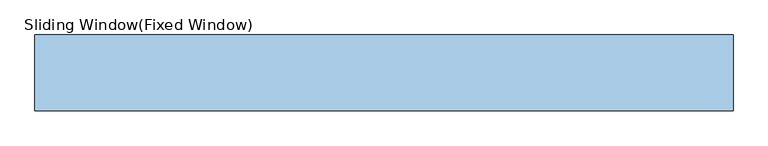
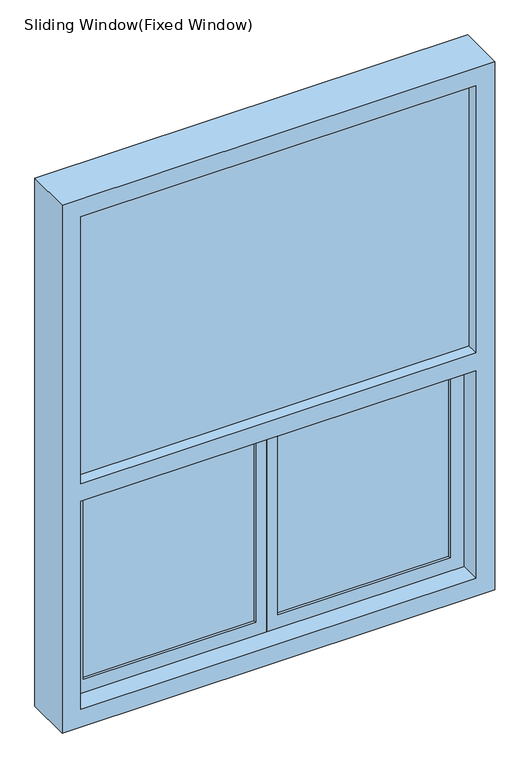
"""IFC4 building model written with IfcOpenShell, lengths in millimetres: window geometry, Sliding Window(Fixed Window) : H_WD_AR_B11_Fix_Sliding_Steel Window_DG_W1400xH1800_AW-1."""

import ifcopenshell
import ifcopenshell.guid

model = None  # the IFC model being written
_history = None  # IfcOwnerHistory: only IFC2X3 demands one
_inside = {}  # id of a spatial element -> (the spatial element, [elements in it])
_under = {}  # id of a project, library or spatial element -> (it, [spatial elements below it])
_declared = {}  # id of a project -> (the project, [libraries it declares])
_typed = {}  # id of a type object -> (the type object, [elements of that type])
_made_of = {}  # id of a material, layer set ... -> (it, [elements and type objects made of it])


def new_model(schema):
    """Start an empty IFC model of exactly this schema.

    Asked for "IFC4X3", IfcOpenShell would pick the latest addendum, in which some entities
    have other attributes; the version numbers below select the first issue.
    IFC2X3 requires an IfcOwnerHistory on every rooted entity: one is made here for all.
    """
    global model, _history
    if schema == "IFC4X3":
        model = ifcopenshell.file(schema_version=(4, 3, 0, 0))
    else:
        model = ifcopenshell.file(schema=schema)
    _inside.clear()
    _under.clear()
    _declared.clear()
    _typed.clear()
    _made_of.clear()
    _history = None
    if model.schema == "IFC2X3":
        org = make("IfcOrganization", Name="unknown")
        user = make(
            "IfcPersonAndOrganization",
            ThePerson=make("IfcPerson", FamilyName="unknown"),
            TheOrganization=org,
        )
        app = make(
            "IfcApplication",
            ApplicationDeveloper=org,
            Version="unknown",
            ApplicationFullName="unknown",
            ApplicationIdentifier="unknown",
        )
        _history = make(
            "IfcOwnerHistory",
            OwningUser=user,
            OwningApplication=app,
            ChangeAction="ADDED",
            CreationDate=0,
        )
    return model


def make(cls, **values):
    """One entity of the class cls with the attributes given. An attribute that is None is left unset."""
    return model.create_entity(
        cls, **{name: value for name, value in values.items() if value is not None}
    )


def rooted(cls, **values):
    """An entity with a GlobalId (a new one), such as an element, a storey or a relation."""
    return make(cls, GlobalId=ifcopenshell.guid.new(), OwnerHistory=_history, **values)


def si_unit(unit_type, name, prefix=None):
    """IfcSIUnit, for example si_unit("LENGTHUNIT", "METRE", prefix="MILLI")."""
    return make("IfcSIUnit", UnitType=unit_type, Prefix=prefix, Name=name)


def assignment(units):
    """IfcUnitAssignment: the units of a project."""
    return None if units is None else make("IfcUnitAssignment", Units=units)


def point(xyz):
    """IfcCartesianPoint."""
    return None if xyz is None else make("IfcCartesianPoint", Coordinates=xyz)


def direction(xyz):
    """IfcDirection."""
    return None if xyz is None else make("IfcDirection", DirectionRatios=xyz)


def frame(location, z_axis=None, x_axis=None):
    """IfcAxis2Placement3D, a coordinate frame: its origin and axes. An axis left out is left unset."""
    return make(
        "IfcAxis2Placement3D",
        Location=point(location),
        Axis=direction(z_axis),
        RefDirection=direction(x_axis),
    )


def origin():
    """The frame at (0, 0, 0) with its axes left unset."""
    return frame((0.0, 0.0, 0.0))


def place(relative_to, where):
    """IfcLocalPlacement: puts the frame where relative to a parent placement (None: the world)."""
    return make(
        "IfcLocalPlacement", PlacementRelTo=relative_to, RelativePlacement=where
    )


def context(
    kind, dimensions, precision=None, world=None, true_north=None, identifier=None
):
    """IfcGeometricRepresentationContext, for example the 3D "Model" context."""
    return make(
        "IfcGeometricRepresentationContext",
        ContextIdentifier=identifier,
        ContextType=kind,
        CoordinateSpaceDimension=dimensions,
        Precision=precision,
        WorldCoordinateSystem=world,
        TrueNorth=true_north,
    )


def project(units=None, contexts=None):
    """IfcProject with its units and contexts."""
    return rooted(
        "IfcProject",
        Name="project",
        RepresentationContexts=contexts,
        UnitsInContext=assignment(units),
    )


def spatial(cls, under=None, at=None, **own):
    """A site, building, storey or space (cls), placed at a placement, below another one or the project."""
    s = rooted(cls, ObjectPlacement=at, **own)
    if under is not None:
        _under.setdefault(under.id(), (under, []))[1].append(s)
    return s


def polyline(points):
    """IfcPolyline through the points."""
    return make("IfcPolyline", Points=[point(p) for p in points])


def outline(outer, holes=None, kind="AREA"):
    """IfcArbitraryClosedProfileDef: a profile drawn as a closed curve; with holes, ...WithVoids."""
    if holes is None:
        return make("IfcArbitraryClosedProfileDef", ProfileType=kind, OuterCurve=outer)
    return make(
        "IfcArbitraryProfileDefWithVoids",
        ProfileType=kind,
        OuterCurve=outer,
        InnerCurves=holes,
    )


def extrude(swept, where, along, depth):
    """IfcExtrudedAreaSolid: the profile swept, set in the frame where, extruded along a direction by depth."""
    return make(
        "IfcExtrudedAreaSolid",
        SweptArea=swept,
        Position=where,
        ExtrudedDirection=direction(along),
        Depth=depth,
    )


def shape(context_of_items, identifier, shape_type, items):
    """IfcShapeRepresentation: the items that make up one representation, for example the "Body"."""
    return make(
        "IfcShapeRepresentation",
        ContextOfItems=context_of_items,
        RepresentationIdentifier=identifier,
        RepresentationType=shape_type,
        Items=items,
    )


def source(mapping_origin, context_of_items, identifier, shape_type, items):
    """IfcRepresentationMap: a shape defined once, which mapped items show again and again."""
    return make(
        "IfcRepresentationMap",
        MappingOrigin=mapping_origin,
        MappedRepresentation=shape(context_of_items, identifier, shape_type, items),
    )


def transform(
    local_origin,
    x_axis=None,
    y_axis=None,
    z_axis=None,
    scale=None,
    scale2=None,
    scale3=None,
    uniform=True,
):
    """IfcCartesianTransformationOperator3D, or its non-uniform kind. x_axis, y_axis, z_axis: its Axis1, 2, 3."""
    if uniform:
        return make(
            "IfcCartesianTransformationOperator3D",
            Axis1=direction(x_axis),
            Axis2=direction(y_axis),
            LocalOrigin=point(local_origin),
            Scale=scale,
            Axis3=direction(z_axis),
        )
    return make(
        "IfcCartesianTransformationOperator3DnonUniform",
        Axis1=direction(x_axis),
        Axis2=direction(y_axis),
        LocalOrigin=point(local_origin),
        Scale=scale,
        Axis3=direction(z_axis),
        Scale2=scale2,
        Scale3=scale3,
    )


def mapped(mapping_source, mapping_target):
    """IfcMappedItem: shows the shape of a source again, moved by a transform."""
    return make(
        "IfcMappedItem", MappingSource=mapping_source, MappingTarget=mapping_target
    )


def made_of(thing, what):
    """Note that an element or type object is made of a material, layer set ...; save() writes the relation."""
    if what is not None:
        _made_of.setdefault(what.id(), (what, []))[1].append(thing)
    return thing


def element(
    cls,
    number,
    at=None,
    inside=None,
    cuts=None,
    type_object=None,
    material=None,
    context=None,
    identifier="Body",
    shape_type=None,
    held_by="IfcProductDefinitionShape",
    body=None,
    shapes=None,
    **own,
):
    """One element of the class cls, such as IfcWall. Its Tag is "e" and its number.

    at: its placement. inside: the storey or other place that contains it. cuts: it is an
    opening in that element (IfcRelVoidsElement). A single representation is given by context,
    identifier, shape_type and body (its items); several are given by shapes. held_by: the class
    of the entity that holds the representations. save() writes the other relations.
    """
    e = rooted(cls, Tag="e%d" % number, ObjectPlacement=at, **own)
    if body is not None:
        shapes = [shape(context, identifier, shape_type, body)]
    if shapes is not None:
        e.Representation = make(held_by, Representations=shapes)
    if inside is not None:
        _inside.setdefault(inside.id(), (inside, []))[1].append(e)
    if cuts is not None:
        rooted(
            "IfcRelVoidsElement", RelatingBuildingElement=cuts, RelatedOpeningElement=e
        )
    if type_object is not None:
        _typed.setdefault(type_object.id(), (type_object, []))[1].append(e)
    return made_of(e, material)


def aggregate(whole, parts):
    """IfcRelAggregates: a whole, such as a stair, and the parts it consists of."""
    return rooted("IfcRelAggregates", RelatingObject=whole, RelatedObjects=parts)


def save(model, path):
    """Write the relations noted so far, then the file.

    IfcRelAggregates (storeys below a building ...), IfcRelContainedInSpatialStructure (elements
    in a storey), IfcRelDefinesByType, IfcRelAssociatesMaterial and IfcRelDeclares: one each for
    every whole, place, type object, material and project.
    """
    for whole, parts in _under.values():
        aggregate(whole, parts)
    for where, things in _inside.values():
        rooted(
            "IfcRelContainedInSpatialStructure",
            RelatedElements=things,
            RelatingStructure=where,
        )
    for kind, things in _typed.values():
        rooted("IfcRelDefinesByType", RelatedObjects=things, RelatingType=kind)
    for what, things in _made_of.values():
        rooted("IfcRelAssociatesMaterial", RelatedObjects=things, RelatingMaterial=what)
    for by, libraries in _declared.values():
        rooted("IfcRelDeclares", RelatingContext=by, RelatedDefinitions=libraries)
    model.write(path)


def sliding_window_fixed_window_7f21aae4(model_context):
    return source(origin(), model_context, "Body", "SweptSolid", [
        extrude(outline(polyline([(2830.0, -690.0), (1050.0, -690.0), (1050.0, 690.0), (2830.0, 690.0), (2830.0, -690.0)]), holes=[polyline([(1810.0, 630.0), (1110.0, 630.0), (1110.0, -630.0), (1810.0, -630.0), (1810.0, 630.0)]), polyline([(1870.0, -630.0), (2770.0, -630.0), (2770.0, 630.0), (1870.0, 630.0), (1870.0, -630.0)])]), frame((0.0, -25.0, 0.0), z_axis=(0.0, 1.0, 0.0), x_axis=(0.0, 0.0, 1.0)), (0.0, 0.0, 1.0), 150.0),
        extrude(outline(polyline([(630.0, 37.0), (630.0, 13.0), (-630.0, 13.0), (-630.0, 37.0), (630.0, 37.0)])), frame((0.0, 0.0, 1870.0), z_axis=(0.0, 0.0, 1.0), x_axis=(1.0, 0.0, 0.0)), (0.0, 0.0, 1.0), 900.0),
        extrude(outline(polyline([(-35.0, 61.0), (-35.0, 49.0), (-585.0, 49.0), (-585.0, 61.0), (-35.0, 61.0)])), frame((0.0, 0.0, 1155.0), z_axis=(0.0, 0.0, 1.0), x_axis=(1.0, 0.0, 0.0)), (0.0, 0.0, 1.0), 610.0),
        extrude(outline(polyline([(1810.0, -630.0), (1110.0, -630.0), (1110.0, 0.0), (1810.0, 0.0), (1810.0, -630.0)]), holes=[polyline([(1765.0, -585.0), (1765.0, -35.0), (1155.0, -35.0), (1155.0, -585.0), (1765.0, -585.0)])]), frame((0.0, 40.0, 0.0), z_axis=(0.0, 1.0, 0.0), x_axis=(0.0, 0.0, 1.0)), (0.0, 0.0, 1.0), 30.0),
        extrude(outline(polyline([(585.0, 61.0), (585.0, 49.0), (35.0, 49.0), (35.0, 61.0), (585.0, 61.0)])), frame((0.0, 0.0, 1155.0), z_axis=(0.0, 0.0, 1.0), x_axis=(1.0, 0.0, 0.0)), (0.0, 0.0, 1.0), 610.0),
        extrude(outline(polyline([(1810.0, 0.0), (1110.0, 0.0), (1110.0, 630.0), (1810.0, 630.0), (1810.0, 0.0)]), holes=[polyline([(1765.0, 35.0), (1765.0, 585.0), (1155.0, 585.0), (1155.0, 35.0), (1765.0, 35.0)])]), frame((0.0, 40.0, 0.0), z_axis=(0.0, 1.0, 0.0), x_axis=(0.0, 0.0, 1.0)), (0.0, 0.0, 1.0), 30.0),
    ])


if __name__ == "__main__":
    model = new_model("IFC4")
    model_context = context("Model", 3, world=origin())
    ifc_project = project(units=[si_unit("LENGTHUNIT", "METRE", prefix="MILLI")], contexts=[model_context])
    site = spatial("IfcSite", under=ifc_project)
    building = spatial("IfcBuilding", under=site)
    placement = place(None, origin())
    sliding_window_fixed_window_shape = sliding_window_fixed_window_7f21aae4(model_context)
    element("IfcWindow", 1, ObjectType="Sliding Window(Fixed Window) : H_WD_AR_B11_Fix_Sliding_Steel Window_DG_W1400xH1800_AW-1", at=placement, inside=building, context=model_context, shape_type="MappedRepresentation", body=[
        mapped(sliding_window_fixed_window_shape, transform((0.0, 0.0, 0.0), x_axis=(1.0, 0.0, 0.0), y_axis=(0.0, 1.0, 0.0), z_axis=(0.0, 0.0, 1.0))),
    ])
    save(model, "model.ifc")

# Revit data of these elements
# Type "Sliding Window(Fixed Window) : H_WD_AR_B11_Fix_Sliding_Steel Window_DG_W1400xH1800_AW-1"
#   Type Mark = "268"
#   Analytic Construction = "<None>"
#   미서기창 높이 = 700 mm
#   Main Window = 1400 mm
#   Height = 1800 mm
#   Mullion Thk = 60 mm
#   Frame = 150 mm
#   Default Sill Height = 1040 mm
#   Width = 1400 mm
#   Define Thermal Properties by = 1
#   Wall Closure = (empty or 0)
# Element 1 (IfcWindow, "Sliding Window(Fixed Window) : H_WD_AR_B11_Fix_Sliding_Steel Window_DG_W1400xH1800_AW-1")
#   Materials on its faces: "00_Metal_Aluminum", "Glass"
# Materials
#   "00_Metal_Aluminum": class "Metal", colour RGB 244 244 244, transparency 0, Description = "Aluminum", Cost = 0, Image = none
#   "Glass": class "Glass", colour RGB 218 227 224, transparency 0.85, Description = "Soda Lime Glass", Cost = 0
